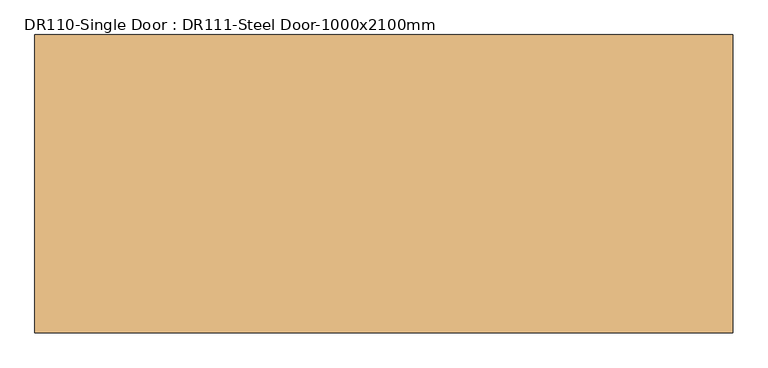
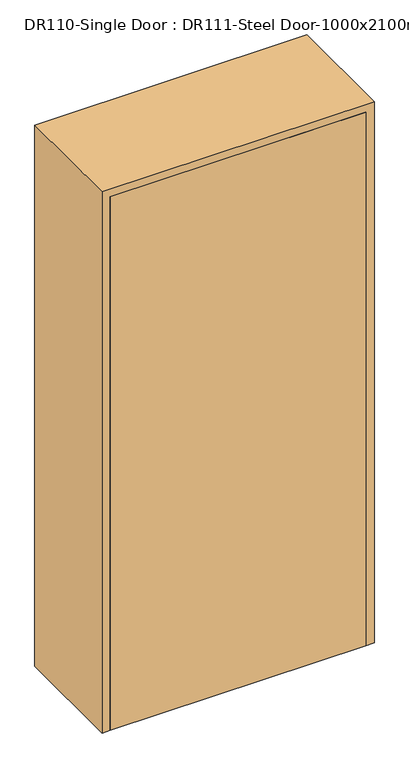
"""IFC4 building model written with IfcOpenShell, lengths in millimetres: door geometry, DR110-Single Door : DR111-Steel Door-1000x2100mm."""

from ifc_helpers import new_model, si_unit, origin, origin_with_axes, place, context, project, spatial, polyline, outline, extrude, faceted_brep, source, transform, mapped, element, save


def dr110_single_door_dr111_steel_door_1000x2100mm_001ab876(model_context):
    return source(origin(), model_context, "Body", "SolidModel", [
        extrude(outline(polyline([(470.0, -213.5), (-470.0, -213.5), (-470.0, -178.5), (470.0, -178.5), (470.0, -213.5)])), origin_with_axes(), (0.0, 0.0, 1.0), 2070.0),
        faceted_brep([(470.0, -213.5, 0.0), (470.0, -178.5, 0.0), (450.0, -178.5, 0.0), (450.0, 178.5, 0.0), (470.0, 178.5, 0.0), (470.0, 213.5, 0.0), (500.0, 213.5, 0.0), (500.0, -213.5, 0.0), (500.0, -213.5, 2100.0), (-500.0, -213.5, 2100.0), (-500.0, -213.5, 0.0), (-470.0, -213.5, 0.0), (-470.0, -213.5, 2070.0), (470.0, -213.5, 2070.0), (500.0, 213.5, 2100.0), (470.0, 213.5, 2070.0), (-470.0, 213.5, 2070.0), (-470.0, 213.5, 0.0), (-500.0, 213.5, 0.0), (-500.0, 213.5, 2100.0), (470.0, 178.5, 2070.0), (450.0, 178.5, 2050.0), (-450.0, 178.5, 2050.0), (-450.0, 178.5, 0.0), (-470.0, 178.5, 0.0), (-470.0, 178.5, 2070.0), (450.0, -178.5, 2050.0), (470.0, -178.5, 2070.0), (-470.0, -178.5, 2070.0), (-470.0, -178.5, 0.0), (-450.0, -178.5, 0.0), (-450.0, -178.5, 2050.0)], [[[0, 1, 2, 3, 4, 5, 6, 7]], [[7, 8, 9, 10, 11, 12, 13, 0]], [[6, 14, 8, 7]], [[5, 15, 16, 17, 18, 19, 14, 6]], [[4, 20, 15, 5]], [[3, 21, 22, 23, 24, 25, 20, 4]], [[2, 26, 21, 3]], [[1, 27, 28, 29, 30, 31, 26, 2]], [[0, 13, 27, 1]], [[12, 11, 29, 28]], [[11, 10, 18, 17, 24, 23, 30, 29]], [[19, 18, 10, 9]], [[25, 24, 17, 16]], [[31, 30, 23, 22]], [[14, 19, 9, 8]], [[20, 25, 16, 15]], [[26, 31, 22, 21]], [[13, 12, 28, 27]]]),
    ])


if __name__ == "__main__":
    model = new_model("IFC4")
    model_context = context("Model", 3, world=origin())
    ifc_project = project(units=[si_unit("LENGTHUNIT", "METRE", prefix="MILLI")], contexts=[model_context])
    site = spatial("IfcSite", under=ifc_project)
    building = spatial("IfcBuilding", under=site)
    placement = place(None, origin())
    dr110_single_door_dr111_steel_door_1000x2100mm_shape = dr110_single_door_dr111_steel_door_1000x2100mm_001ab876(model_context)
    element("IfcDoor", 1, ObjectType="DR110-Single Door : DR111-Steel Door-1000x2100mm", at=placement, inside=building, context=model_context, shape_type="MappedRepresentation", body=[
        mapped(dr110_single_door_dr111_steel_door_1000x2100mm_shape, transform((0.0, 0.0, 0.0), x_axis=(1.0, 0.0, 0.0), y_axis=(0.0, 1.0, 0.0), z_axis=(0.0, 0.0, 1.0))),
    ])
    save(model, "model.ifc")

# Revit data of these elements
# Type "DR110-Single Door : DR111-Steel Door-1000x2100mm"
#   Description = "DSDSSD"
#   Type Mark = "SD"
#   Analytic Construction = "<None>"
#   프레임 투영 외부. = 25 mm
#   프레임 투영 내부. = 25 mm
#   프레임 폭 = 75 mm
#   Height = 2100 mm
#   Width = 1000 mm
#   Define Thermal Properties by = 1
#   문 패널 = SD1 문 패널
#   문 프레임 = A04AQ098-00002_Steel Door_non FP_single
#   Function = (empty or 0)
#   Wall Closure = (empty or 0)
# Element 1 (IfcDoor, "DR110-Single Door : DR111-Steel Door-1000x2100mm")
#   Materials on its faces: "A04AQ098-00002_Steel Door_non FP_single", "SD1 문 패널"
# Materials
#   "SD1 문 패널": class "금속", colour RGB 247 247 247, transparency 0, Description = "STEEL DOOR (1000Wx2100H)"
#   "A04AQ098-00002_Steel Door_non FP_single": class "금속", colour RGB 247 247 247, transparency 0, Description = "Steel Door", W00) Work Master Code = "A04AQ098-00002", W01) Work Master_Lv1 = "Finishing Work", W02) Work Master_Lv2 = "Door & Window Work", W03) Work Master_Spec.1 = "Steel Door w/ Steel Frame", W04) Work Master_Spec.2 = "Fire Protective Rating: N/A, Single Door", W05) Work Master_Spec.3 = "w/ Hardware & Accessories", Cost = 0
